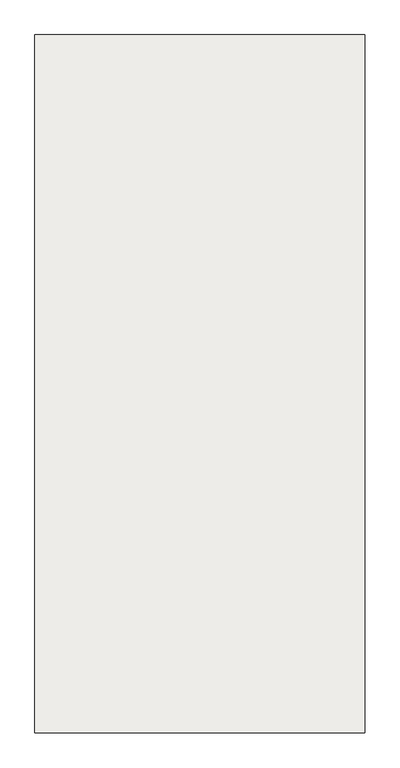
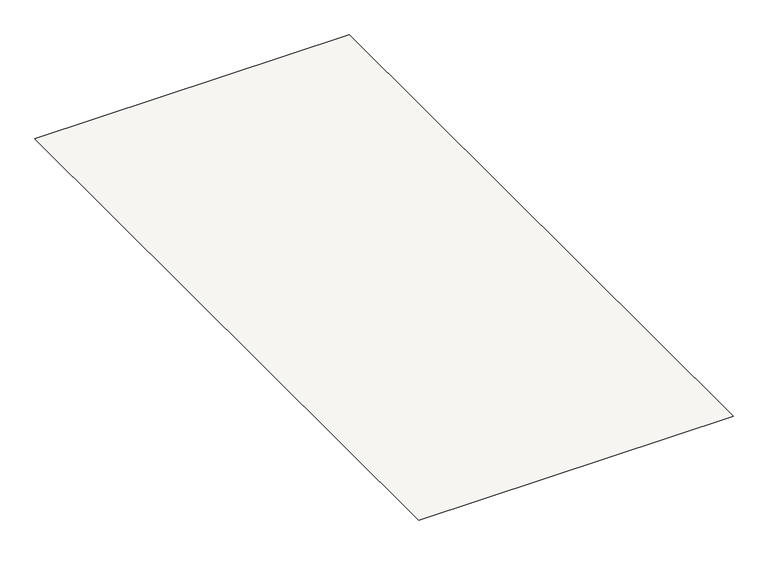
"""IFC4 building model written with IfcOpenShell, lengths in millimetres: slab geometry, EQUIMENT FDN.1 : FTS211_EF_EF1."""

import ifcopenshell
import ifcopenshell.guid

model = None  # the IFC model being written
_history = None  # IfcOwnerHistory: only IFC2X3 demands one
_inside = {}  # id of a spatial element -> (the spatial element, [elements in it])
_under = {}  # id of a project, library or spatial element -> (it, [spatial elements below it])
_declared = {}  # id of a project -> (the project, [libraries it declares])
_typed = {}  # id of a type object -> (the type object, [elements of that type])
_made_of = {}  # id of a material, layer set ... -> (it, [elements and type objects made of it])


def new_model(schema):
    """Start an empty IFC model of exactly this schema.

    Asked for "IFC4X3", IfcOpenShell would pick the latest addendum, in which some entities
    have other attributes; the version numbers below select the first issue.
    IFC2X3 requires an IfcOwnerHistory on every rooted entity: one is made here for all.
    """
    global model, _history
    if schema == "IFC4X3":
        model = ifcopenshell.file(schema_version=(4, 3, 0, 0))
    else:
        model = ifcopenshell.file(schema=schema)
    _inside.clear()
    _under.clear()
    _declared.clear()
    _typed.clear()
    _made_of.clear()
    _history = None
    if model.schema == "IFC2X3":
        org = make("IfcOrganization", Name="unknown")
        user = make(
            "IfcPersonAndOrganization",
            ThePerson=make("IfcPerson", FamilyName="unknown"),
            TheOrganization=org,
        )
        app = make(
            "IfcApplication",
            ApplicationDeveloper=org,
            Version="unknown",
            ApplicationFullName="unknown",
            ApplicationIdentifier="unknown",
        )
        _history = make(
            "IfcOwnerHistory",
            OwningUser=user,
            OwningApplication=app,
            ChangeAction="ADDED",
            CreationDate=0,
        )
    return model


def make(cls, **values):
    """One entity of the class cls with the attributes given. An attribute that is None is left unset."""
    return model.create_entity(
        cls, **{name: value for name, value in values.items() if value is not None}
    )


def rooted(cls, **values):
    """An entity with a GlobalId (a new one), such as an element, a storey or a relation."""
    return make(cls, GlobalId=ifcopenshell.guid.new(), OwnerHistory=_history, **values)


def si_unit(unit_type, name, prefix=None):
    """IfcSIUnit, for example si_unit("LENGTHUNIT", "METRE", prefix="MILLI")."""
    return make("IfcSIUnit", UnitType=unit_type, Prefix=prefix, Name=name)


def assignment(units):
    """IfcUnitAssignment: the units of a project."""
    return None if units is None else make("IfcUnitAssignment", Units=units)


def point(xyz):
    """IfcCartesianPoint."""
    return None if xyz is None else make("IfcCartesianPoint", Coordinates=xyz)


def direction(xyz):
    """IfcDirection."""
    return None if xyz is None else make("IfcDirection", DirectionRatios=xyz)


def frame(location, z_axis=None, x_axis=None):
    """IfcAxis2Placement3D, a coordinate frame: its origin and axes. An axis left out is left unset."""
    return make(
        "IfcAxis2Placement3D",
        Location=point(location),
        Axis=direction(z_axis),
        RefDirection=direction(x_axis),
    )


def origin():
    """The frame at (0, 0, 0) with its axes left unset."""
    return frame((0.0, 0.0, 0.0))


def place(relative_to, where):
    """IfcLocalPlacement: puts the frame where relative to a parent placement (None: the world)."""
    return make(
        "IfcLocalPlacement", PlacementRelTo=relative_to, RelativePlacement=where
    )


def context(
    kind, dimensions, precision=None, world=None, true_north=None, identifier=None
):
    """IfcGeometricRepresentationContext, for example the 3D "Model" context."""
    return make(
        "IfcGeometricRepresentationContext",
        ContextIdentifier=identifier,
        ContextType=kind,
        CoordinateSpaceDimension=dimensions,
        Precision=precision,
        WorldCoordinateSystem=world,
        TrueNorth=true_north,
    )


def project(units=None, contexts=None):
    """IfcProject with its units and contexts."""
    return rooted(
        "IfcProject",
        Name="project",
        RepresentationContexts=contexts,
        UnitsInContext=assignment(units),
    )


def spatial(cls, under=None, at=None, **own):
    """A site, building, storey or space (cls), placed at a placement, below another one or the project."""
    s = rooted(cls, ObjectPlacement=at, **own)
    if under is not None:
        _under.setdefault(under.id(), (under, []))[1].append(s)
    return s


def faces_of(points, faces, orient=None, outer=None):
    """IfcFace entities. A face is a list of loops; a loop is a list of indices into points, from 0.

    orient and outer hold one flag for each loop. By default every Orientation is true, the
    first loop of a face is its IfcFaceOuterBound and the others are IfcFaceBound.
    """
    made = []
    for i, loops in enumerate(faces):
        bounds = []
        for j, loop in enumerate(loops):
            is_outer = j == 0 if outer is None else outer[i][j]
            bounds.append(
                make(
                    "IfcFaceOuterBound" if is_outer else "IfcFaceBound",
                    Bound=make("IfcPolyLoop", Polygon=[points[k] for k in loop]),
                    Orientation=True if orient is None else orient[i][j],
                )
            )
        made.append(make("IfcFace", Bounds=bounds))
    return made


def faceted_brep(points, faces, orient=None, outer=None, voids=None):
    """IfcFacetedBrep: a solid bounded by flat faces; with voids (closed shells), ...WithVoids."""
    shared = [point(p) for p in points]
    hull = make("IfcClosedShell", CfsFaces=faces_of(shared, faces, orient, outer))
    if voids is None:
        return make("IfcFacetedBrep", Outer=hull)
    return make(
        "IfcFacetedBrepWithVoids",
        Outer=hull,
        Voids=[
            make(cls, CfsFaces=faces_of(shared, fs, o, b)) for cls, fs, o, b in voids
        ],
    )


def shape(context_of_items, identifier, shape_type, items):
    """IfcShapeRepresentation: the items that make up one representation, for example the "Body"."""
    return make(
        "IfcShapeRepresentation",
        ContextOfItems=context_of_items,
        RepresentationIdentifier=identifier,
        RepresentationType=shape_type,
        Items=items,
    )


def source(mapping_origin, context_of_items, identifier, shape_type, items):
    """IfcRepresentationMap: a shape defined once, which mapped items show again and again."""
    return make(
        "IfcRepresentationMap",
        MappingOrigin=mapping_origin,
        MappedRepresentation=shape(context_of_items, identifier, shape_type, items),
    )


def transform(
    local_origin,
    x_axis=None,
    y_axis=None,
    z_axis=None,
    scale=None,
    scale2=None,
    scale3=None,
    uniform=True,
):
    """IfcCartesianTransformationOperator3D, or its non-uniform kind. x_axis, y_axis, z_axis: its Axis1, 2, 3."""
    if uniform:
        return make(
            "IfcCartesianTransformationOperator3D",
            Axis1=direction(x_axis),
            Axis2=direction(y_axis),
            LocalOrigin=point(local_origin),
            Scale=scale,
            Axis3=direction(z_axis),
        )
    return make(
        "IfcCartesianTransformationOperator3DnonUniform",
        Axis1=direction(x_axis),
        Axis2=direction(y_axis),
        LocalOrigin=point(local_origin),
        Scale=scale,
        Axis3=direction(z_axis),
        Scale2=scale2,
        Scale3=scale3,
    )


def mapped(mapping_source, mapping_target):
    """IfcMappedItem: shows the shape of a source again, moved by a transform."""
    return make(
        "IfcMappedItem", MappingSource=mapping_source, MappingTarget=mapping_target
    )


def made_of(thing, what):
    """Note that an element or type object is made of a material, layer set ...; save() writes the relation."""
    if what is not None:
        _made_of.setdefault(what.id(), (what, []))[1].append(thing)
    return thing


def element(
    cls,
    number,
    at=None,
    inside=None,
    cuts=None,
    type_object=None,
    material=None,
    context=None,
    identifier="Body",
    shape_type=None,
    held_by="IfcProductDefinitionShape",
    body=None,
    shapes=None,
    **own,
):
    """One element of the class cls, such as IfcWall. Its Tag is "e" and its number.

    at: its placement. inside: the storey or other place that contains it. cuts: it is an
    opening in that element (IfcRelVoidsElement). A single representation is given by context,
    identifier, shape_type and body (its items); several are given by shapes. held_by: the class
    of the entity that holds the representations. save() writes the other relations.
    """
    e = rooted(cls, Tag="e%d" % number, ObjectPlacement=at, **own)
    if body is not None:
        shapes = [shape(context, identifier, shape_type, body)]
    if shapes is not None:
        e.Representation = make(held_by, Representations=shapes)
    if inside is not None:
        _inside.setdefault(inside.id(), (inside, []))[1].append(e)
    if cuts is not None:
        rooted(
            "IfcRelVoidsElement", RelatingBuildingElement=cuts, RelatedOpeningElement=e
        )
    if type_object is not None:
        _typed.setdefault(type_object.id(), (type_object, []))[1].append(e)
    return made_of(e, material)


def aggregate(whole, parts):
    """IfcRelAggregates: a whole, such as a stair, and the parts it consists of."""
    return rooted("IfcRelAggregates", RelatingObject=whole, RelatedObjects=parts)


def save(model, path):
    """Write the relations noted so far, then the file.

    IfcRelAggregates (storeys below a building ...), IfcRelContainedInSpatialStructure (elements
    in a storey), IfcRelDefinesByType, IfcRelAssociatesMaterial and IfcRelDeclares: one each for
    every whole, place, type object, material and project.
    """
    for whole, parts in _under.values():
        aggregate(whole, parts)
    for where, things in _inside.values():
        rooted(
            "IfcRelContainedInSpatialStructure",
            RelatedElements=things,
            RelatingStructure=where,
        )
    for kind, things in _typed.values():
        rooted("IfcRelDefinesByType", RelatedObjects=things, RelatingType=kind)
    for what, things in _made_of.values():
        rooted("IfcRelAssociatesMaterial", RelatedObjects=things, RelatingMaterial=what)
    for by, libraries in _declared.values():
        rooted("IfcRelDeclares", RelatingContext=by, RelatedDefinitions=libraries)
    model.write(path)


def slab_9a1243d7(model_context):
    return source(origin(), model_context, "Body", "Brep", [
        faceted_brep([(48394.0, 29249.5208589, 199.9720055), (48394.0, 25149.5208589, 199.9720055), (46794.0, 25149.5208589, 199.9720055), (46794.0, 29249.5208589, 199.9720055), (46474.0, 29569.5208589, 399.9720055), (48714.0, 29569.5208589, 399.9720055), (46474.0, 24829.5208589, 399.9720055), (48714.0, 24829.5208589, 399.9720055)], [[[0, 1, 2, 3]], [[0, 3, 4, 5]], [[3, 2, 6, 4]], [[2, 1, 7, 6]], [[1, 0, 5, 7]], [[5, 4, 6, 7]]]),
    ])


if __name__ == "__main__":
    model = new_model("IFC4")
    model_context = context("Model", 3, world=origin())
    ifc_project = project(units=[si_unit("LENGTHUNIT", "METRE", prefix="MILLI")], contexts=[model_context])
    site = spatial("IfcSite", under=ifc_project)
    building = spatial("IfcBuilding", under=site)
    placement = place(None, origin())
    slab_shape = slab_9a1243d7(model_context)
    element("IfcSlab", 1, ObjectType="EQUIMENT FDN.1 : FTS211_EF_EF1", at=placement, inside=building, context=model_context, shape_type="MappedRepresentation", body=[
        mapped(slab_shape, transform((0.0, 0.0, 0.0), x_axis=(1.0, 0.0, 0.0), y_axis=(0.0, 1.0, 0.0), z_axis=(0.0, 0.0, 1.0))),
    ])
    save(model, "model.ifc")

# Revit data of these elements
# Element 1 (IfcSlab, "EQUIMENT FDN.1 : FTS211_EF_EF1")
#   Materials on its faces: "A03AD032-00010_Structural Concrete_UG_20-24MPa"
# Materials
#   "A03AD032-00010_Structural Concrete_UG_20-24MPa": class "Concrete", colour RGB 176 176 176, transparency 0, Keynote = "09910.A1", Description = "Substructure Concrete / Cement Type-1 / 24MPa", Cost = 0
